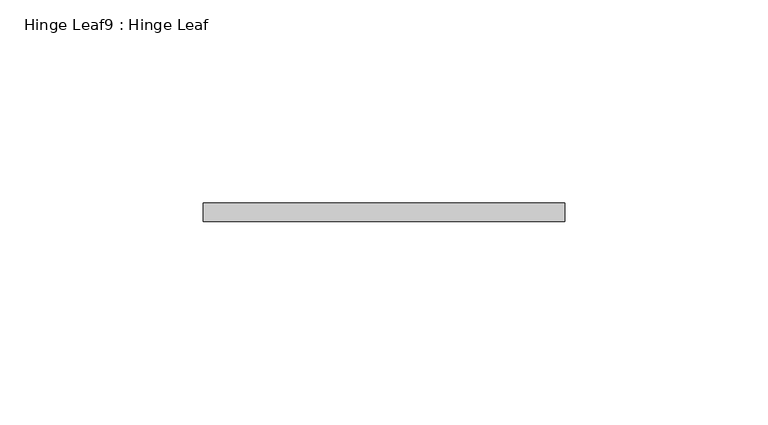
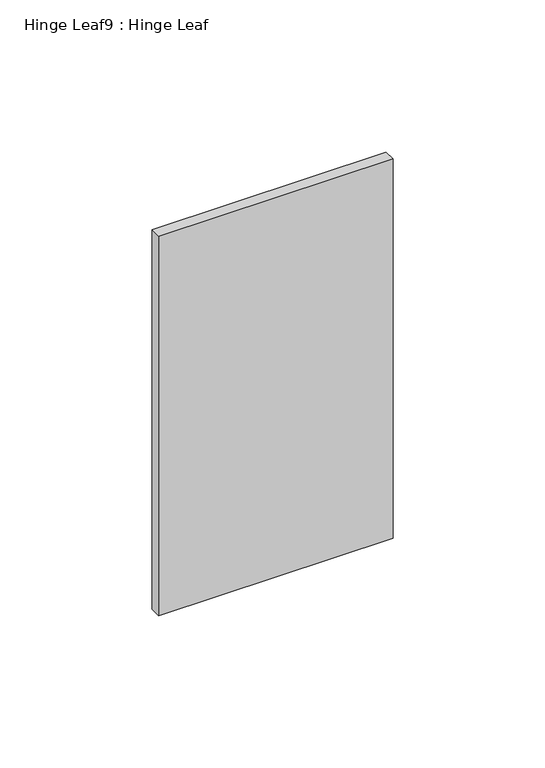
"""IFC4 building model written with IfcOpenShell, lengths in millimetres: proxy geometry, Hinge Leaf9 : Hinge Leaf."""

from ifc_helpers import new_model, si_unit, frame, origin, place, context, project, spatial, polyline, outline, extrude, source, transform, mapped, element, save


def hinge_leaf9_hinge_leaf_49d9ed16(model_context):
    return source(origin(), model_context, "Body", "SweptSolid", [
        extrude(outline(polyline([(587327.7934739, -533988.7163841), (587327.7934739, -533984.1443841), (587416.6934739, -533984.1443841), (587416.6934739, -533988.7163841), (587327.7934739, -533988.7163841)])), frame((0.0, 0.0, 1936.75), z_axis=(0.0, 0.0, 1.0), x_axis=(1.0, 0.0, 0.0)), (0.0, 0.0, 1.0), 152.4),
    ])


if __name__ == "__main__":
    model = new_model("IFC4")
    model_context = context("Model", 3, world=origin())
    ifc_project = project(units=[si_unit("LENGTHUNIT", "METRE", prefix="MILLI")], contexts=[model_context])
    site = spatial("IfcSite", under=ifc_project)
    building = spatial("IfcBuilding", under=site)
    placement = place(None, origin())
    hinge_leaf9_hinge_leaf_shape = hinge_leaf9_hinge_leaf_49d9ed16(model_context)
    element("IfcBuildingElementProxy", 1, Name="Hinge Leaf9 : Hinge Leaf", ObjectType="Hinge Leaf9 : Hinge Leaf", at=placement, inside=building, context=model_context, shape_type="MappedRepresentation", body=[
        mapped(hinge_leaf9_hinge_leaf_shape, transform((0.0, 0.0, 0.0), x_axis=(1.0, 0.0, 0.0), y_axis=(0.0, 1.0, 0.0), z_axis=(0.0, 0.0, 1.0))),
    ])
    save(model, "model.ifc")

# Revit data of these elements
# Element 1 (IfcBuildingElementProxy, "Hinge Leaf9 : Hinge Leaf")
#   Materials on its faces: "6\"X6\" WELD-ON STL BUTT HINGE"
# Materials
#   "6\"X6\" WELD-ON STL BUTT HINGE": class "Metal", colour RGB 189 187 185, transparency 0, Description = "Carbon steel", Cost = 0
